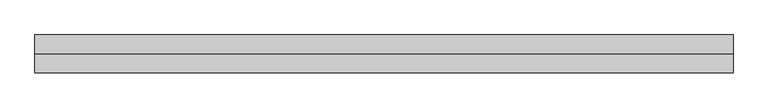
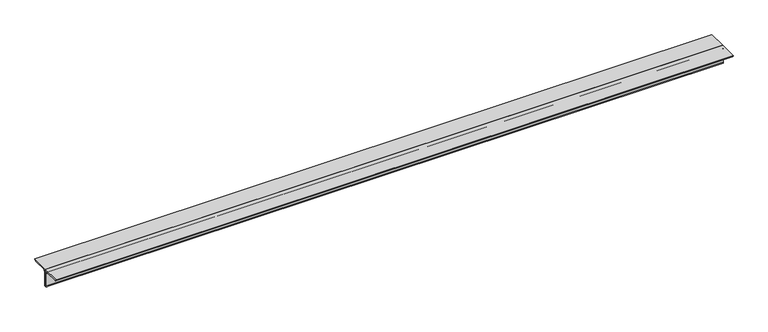
"""IFC4 building model written with IfcOpenShell, lengths in millimetres: member geometry, 0123_Steel Framing_2Ls-KSD3502 : H_SB_AR_S03_2Ls-130x130x12_HBR4."""

from ifc_helpers import new_model, si_unit, point, frame, frame_2d, origin, place, context, project, spatial, polyline, circle_curve, trimmed, segment, composite_curve, outline, extrude, source, transform, mapped, element, save


def member_ef68aef1(model_context):
    return source(origin(), model_context, "Body", "SweptSolid", [
        extrude(outline(composite_curve([segment(polyline([(0.0, 36.4), (130.0, 36.4)]), True, "CONTINUOUS"), segment(trimmed(circle_curve(frame_2d((118.0, 36.4)), 12.0), [point((130.0, 36.4))], [point((118.0, 24.4))], False, "CARTESIAN"), True, "CONTINUOUS"), segment(polyline([(118.0, 24.4), (24.0, 24.4)]), True, "CONTINUOUS"), segment(trimmed(circle_curve(frame_2d((24.0, 12.4)), 12.0), [point((24.0, 24.4))], [point((12.0, 12.4))], True, "CARTESIAN"), True, "CONTINUOUS"), segment(polyline([(12.0, 12.4), (12.0, -81.6)]), True, "CONTINUOUS"), segment(trimmed(circle_curve(frame_2d((0.0, -81.6)), 12.0), [point((12.0, -81.6))], [point((0.0, -93.6))], False, "CARTESIAN"), True, "CONTINUOUS"), segment(polyline([(0.0, -93.6), (0.0, 36.4)]), True, "CONTINUOUS")], self_intersect=False)), frame((-2238.4043387, 0.0, 0.0), z_axis=(1.0, 0.0, 0.0), x_axis=(0.0, 1.0, 0.0)), (0.0, 0.0, 1.0), 4798.1465182),
        extrude(outline(composite_curve([segment(polyline([(0.0, 36.4), (0.0, -93.6)]), True, "CONTINUOUS"), segment(trimmed(circle_curve(frame_2d((0.0, -81.6)), 12.0), [point((0.0, -93.6))], [point((-12.0, -81.6))], False, "CARTESIAN"), True, "CONTINUOUS"), segment(polyline([(-12.0, -81.6), (-12.0, 12.4)]), True, "CONTINUOUS"), segment(trimmed(circle_curve(frame_2d((-24.0, 12.4)), 12.0), [point((-12.0, 12.4))], [point((-24.0, 24.4))], True, "CARTESIAN"), True, "CONTINUOUS"), segment(polyline([(-24.0, 24.4), (-118.0, 24.4)]), True, "CONTINUOUS"), segment(trimmed(circle_curve(frame_2d((-118.0, 36.4)), 12.0), [point((-118.0, 24.4))], [point((-130.0, 36.4))], False, "CARTESIAN"), True, "CONTINUOUS"), segment(polyline([(-130.0, 36.4), (0.0, 36.4)]), True, "CONTINUOUS")], self_intersect=False)), frame((-2238.4043387, 0.0, 0.0), z_axis=(1.0, 0.0, 0.0), x_axis=(0.0, 1.0, 0.0)), (0.0, 0.0, 1.0), 4798.1465182),
    ])


if __name__ == "__main__":
    model = new_model("IFC4")
    model_context = context("Model", 3, world=origin())
    ifc_project = project(units=[si_unit("LENGTHUNIT", "METRE", prefix="MILLI")], contexts=[model_context])
    site = spatial("IfcSite", under=ifc_project)
    building = spatial("IfcBuilding", under=site)
    placement = place(None, origin())
    member_shape = member_ef68aef1(model_context)
    element("IfcMember", 1, ObjectType="0123_Steel Framing_2Ls-KSD3502 : H_SB_AR_S03_2Ls-130x130x12_HBR4", at=placement, inside=building, context=model_context, shape_type="MappedRepresentation", body=[
        mapped(member_shape, transform((0.0, 0.0, 0.0), x_axis=(1.0, 0.0, 0.0), y_axis=(0.0, 1.0, 0.0), z_axis=(0.0, 0.0, 1.0))),
    ])
    save(model, "model.ifc")

# Revit data of these elements
# Type "0123_Steel Framing_2Ls-KSD3502 : H_SB_AR_S03_2Ls-130x130x12_HBR4"
#   Assembly Code = "B10"
#   Legs = "SLBB"
#   W = 8.97
#   Perimeter = 1.04 m²/m
#   Nominal Weight = 46.80 kgf/m
#   Length [instance default] = 1000 mm
#   Space = 0 mm
#   b = 130 mm
#   d = 130 mm
#   t = 12 mm
#   y = 36.4 mm
#   A = 0.005952 m²
#   Structural Material [instance default] = Steel ASTM A36
# Element 1 (IfcMember, "0123_Steel Framing_2Ls-KSD3502 : H_SB_AR_S03_2Ls-130x130x12_HBR4")
#   Structural Material = Steel, 45-345
#   Materials on its faces: "Steel, 45-345"
# Materials
#   "Steel ASTM A36": class "Metal", colour RGB 199 199 199, transparency 0, Description = "Structural steel, ASTM A36 Grade B, mill finish", Cost = 0
#   "Steel, 45-345": class "Metal", colour RGB 189 187 185, transparency 0, Description = "Steel 345 MPa", Cost = 0
